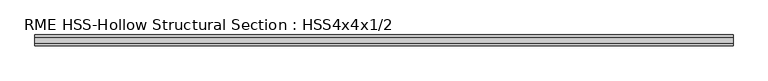
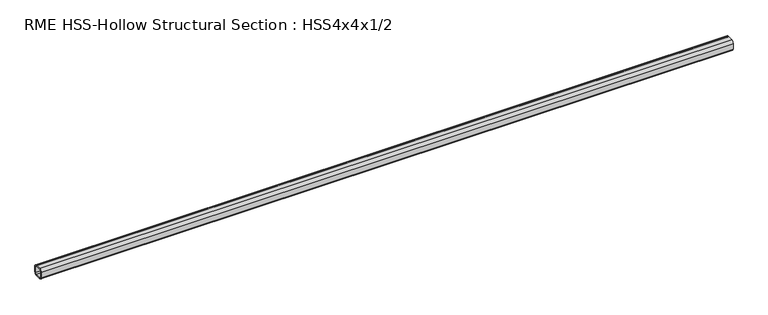
"""IFC4 building model written with IfcOpenShell, lengths in millimetres: member geometry, RME HSS-Hollow Structural Section : HSS4x4x1/2."""

from ifc_helpers import new_model, si_unit, point, frame, frame_2d, origin, place, context, project, spatial, polyline, circle_curve, trimmed, segment, composite_curve, outline, extrude, source, transform, mapped, element, save


def rme_hss_hollow_structural_section_hss4x4x1_2_f373f2e3(model_context):
    return source(origin(), model_context, "Body", "SweptSolid", [
        extrude(outline(composite_curve([segment(polyline([(50.8, 27.178), (50.8, -27.178)]), True, "CONTINUOUS"), segment(trimmed(circle_curve(frame_2d((27.178, -27.178)), 23.622), [point((50.8, -27.178))], [point((27.178, -50.8))], False, "CARTESIAN"), True, "CONTINUOUS"), segment(polyline([(27.178, -50.8), (-27.178, -50.8)]), True, "CONTINUOUS"), segment(trimmed(circle_curve(frame_2d((-27.178, -27.178)), 23.622), [point((-27.178, -50.8))], [point((-50.8, -27.178))], False, "CARTESIAN"), True, "CONTINUOUS"), segment(polyline([(-50.8, -27.178), (-50.8, 27.178)]), True, "CONTINUOUS"), segment(trimmed(circle_curve(frame_2d((-27.178, 27.178)), 23.622), [point((-50.8, 27.178))], [point((-27.178, 50.8))], False, "CARTESIAN"), True, "CONTINUOUS"), segment(polyline([(-27.178, 50.8), (27.178, 50.8)]), True, "CONTINUOUS"), segment(trimmed(circle_curve(frame_2d((27.178, 27.178)), 23.622), [point((27.178, 50.8))], [point((50.8, 27.178))], False, "CARTESIAN"), True, "CONTINUOUS")], self_intersect=False), holes=[composite_curve([segment(trimmed(circle_curve(frame_2d((-27.178, 27.178)), 11.811), [point((-27.178, 38.989))], [point((-38.989, 27.178))], True, "CARTESIAN"), True, "CONTINUOUS"), segment(polyline([(-38.989, 27.178), (-38.989, -27.178)]), True, "CONTINUOUS"), segment(trimmed(circle_curve(frame_2d((-27.178, -27.178)), 11.811), [point((-38.989, -27.178))], [point((-27.178, -38.989))], True, "CARTESIAN"), True, "CONTINUOUS"), segment(polyline([(-27.178, -38.989), (27.178, -38.989)]), True, "CONTINUOUS"), segment(trimmed(circle_curve(frame_2d((27.178, -27.178)), 11.811), [point((27.178, -38.989))], [point((38.989, -27.178))], True, "CARTESIAN"), True, "CONTINUOUS"), segment(polyline([(38.989, -27.178), (38.989, 27.178)]), True, "CONTINUOUS"), segment(trimmed(circle_curve(frame_2d((27.178, 27.178)), 11.811), [point((38.989, 27.178))], [point((27.178, 38.989))], True, "CARTESIAN"), True, "CONTINUOUS"), segment(polyline([(27.178, 38.989), (-27.178, 38.989)]), True, "CONTINUOUS")], self_intersect=False)]), frame((-3236.5175113, 0.0, 0.0), z_axis=(1.0, 0.0, 0.0), x_axis=(0.0, 1.0, 0.0)), (0.0, 0.0, 1.0), 6474.421969),
    ])


if __name__ == "__main__":
    model = new_model("IFC4")
    model_context = context("Model", 3, world=origin())
    ifc_project = project(units=[si_unit("LENGTHUNIT", "METRE", prefix="MILLI")], contexts=[model_context])
    site = spatial("IfcSite", under=ifc_project)
    building = spatial("IfcBuilding", under=site)
    placement = place(None, origin())
    rme_hss_hollow_structural_section_hss4x4x1_2_shape = rme_hss_hollow_structural_section_hss4x4x1_2_f373f2e3(model_context)
    element("IfcMember", 1, ObjectType="RME HSS-Hollow Structural Section : HSS4x4x1/2", at=placement, inside=building, context=model_context, shape_type="MappedRepresentation", body=[
        mapped(rme_hss_hollow_structural_section_hss4x4x1_2_shape, transform((0.0, 0.0, 0.0), x_axis=(1.0, 0.0, 0.0), y_axis=(0.0, 1.0, 0.0), z_axis=(0.0, 0.0, 1.0))),
    ])
    save(model, "model.ifc")

# Revit data of these elements
# Type "RME HSS-Hollow Structural Section : HSS4x4x1/2"
#   Nominal Size = "HSS6x4"
#   Assembly Code = "B10"
#   Shape = "Square"
#   W = 21.5
#   Start Extension Calculation [instance default] = 10' - 0"
#   Start Extension [instance default] = -0' - 0 1/2"
#   End Extension Calculation [instance default] = 10' - 0"
#   End Extension [instance default] = -0' - 0 1/2"
#   Ht = 0' - 4"
#   Length [instance default] = 5' - 0"
#   b = 0' - 4"
#   kr = 0' - 0.93"
#   t = 0' - 0.465"
#   A = 0.0418056 SF
#   Structural Material [instance default] = Metal - Steel - ASTM A500 - Grade B - Rectangular and Square
# Element 1 (IfcMember, "RME HSS-Hollow Structural Section : HSS4x4x1/2")
#   Length = 23' - 0.59752"
#   Structural Material = Metal - Steel - ASTM A992
#   Materials on its faces: "Metal - Steel - ASTM A992"
# Materials
#   "Metal - Steel - ASTM A500 - Grade B - Rectangular and Square": class "Metal", colour RGB 255 128 0, transparency 0
#   "Metal - Steel - ASTM A992": class "Metal", colour RGB 255 128 0, transparency 0
